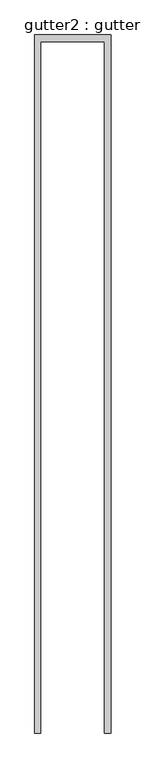
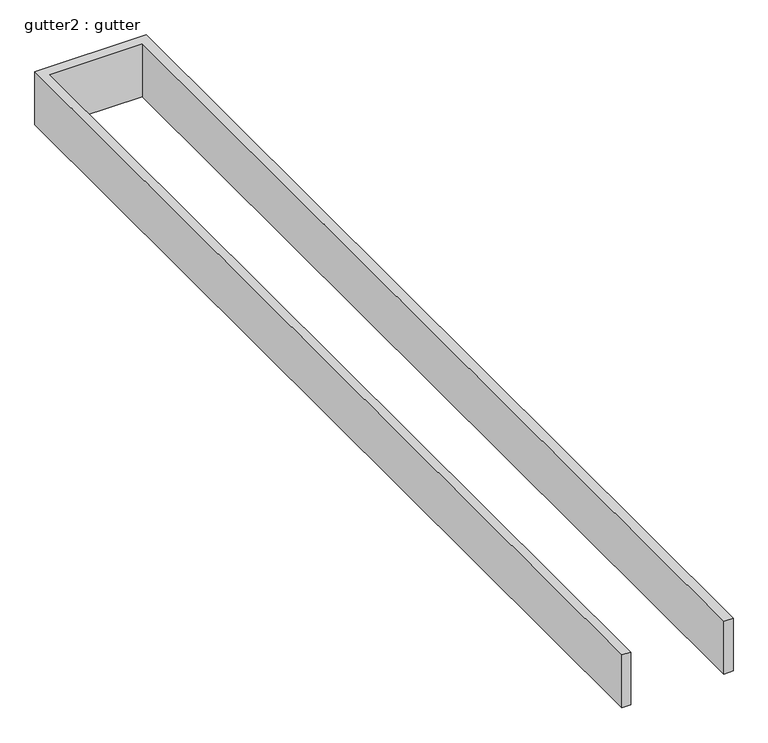
"""IFC4 building model written with IfcOpenShell, lengths in millimetres: proxy geometry, gutter2 : gutter."""

from ifc_helpers import new_model, si_unit, frame, origin, place, context, project, spatial, polyline, outline, extrude, source, transform, mapped, element, save


def gutter2_gutter_d7d01a53(model_context):
    return source(origin(), model_context, "Body", "SweptSolid", [
        extrude(outline(polyline([(29060.890133, 2515.8615366), (29060.890133, 8064.3148819), (29667.201408, 8064.3148819), (29667.201408, 2515.8615366), (29616.401408, 2515.8615366), (29616.401408, 8009.9148819), (29107.4271173, 8009.9148819), (29107.4271173, 2515.8615366), (29060.890133, 2515.8615366)])), frame((0.0, 0.0, 2832.1), z_axis=(0.0, 0.0, 1.0), x_axis=(1.0, 0.0, 0.0)), (0.0, 0.0, 1.0), 304.8),
    ])


if __name__ == "__main__":
    model = new_model("IFC4")
    model_context = context("Model", 3, world=origin())
    ifc_project = project(units=[si_unit("LENGTHUNIT", "METRE", prefix="MILLI")], contexts=[model_context])
    site = spatial("IfcSite", under=ifc_project)
    building = spatial("IfcBuilding", under=site)
    placement = place(None, origin())
    gutter2_gutter_shape = gutter2_gutter_d7d01a53(model_context)
    element("IfcBuildingElementProxy", 1, Name="gutter2 : gutter", ObjectType="gutter2 : gutter", at=placement, inside=building, context=model_context, shape_type="MappedRepresentation", body=[
        mapped(gutter2_gutter_shape, transform((0.0, 0.0, 0.0), x_axis=(1.0, 0.0, 0.0), y_axis=(0.0, 1.0, 0.0), z_axis=(0.0, 0.0, 1.0))),
    ])
    save(model, "model.ifc")
